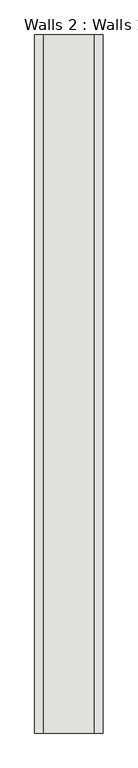
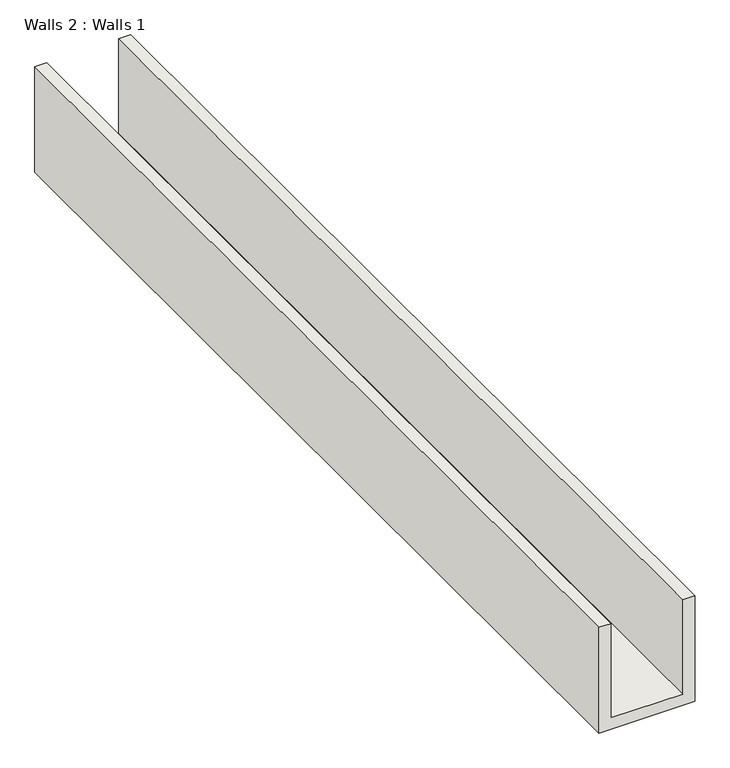
"""IFC4 building model written with IfcOpenShell, lengths in millimetres: wall geometry, Walls 2 : Walls 1."""

from ifc_helpers import new_model, si_unit, frame, origin, place, context, project, spatial, polyline, outline, extrude, source, transform, mapped, element, save


def walls_2_walls_1_c83e6538(model_context):
    return source(origin(), model_context, "Body", "SweptSolid", [
        extrude(outline(polyline([(2794.0, -1677.3168771), (3149.6, -1677.3168771), (3149.6, -1715.4168771), (2832.1, -1715.4168771), (2832.1, -1944.0168771), (3149.6, -1944.0168771), (3149.6, -1982.1168771), (2794.0, -1982.1168771), (2794.0, -1677.3168771)])), frame((0.0, -3023.5771465, 0.0), z_axis=(0.0, 1.0, 0.0), x_axis=(0.0, 0.0, 1.0)), (0.0, 0.0, 1.0), 3114.7191067),
    ])


if __name__ == "__main__":
    model = new_model("IFC4")
    model_context = context("Model", 3, world=origin())
    ifc_project = project(units=[si_unit("LENGTHUNIT", "METRE", prefix="MILLI")], contexts=[model_context])
    site = spatial("IfcSite", under=ifc_project)
    building = spatial("IfcBuilding", under=site)
    placement = place(None, origin())
    walls_2_walls_1_shape = walls_2_walls_1_c83e6538(model_context)
    element("IfcWall", 1, ObjectType="Walls 2 : Walls 1", at=placement, inside=building, context=model_context, shape_type="MappedRepresentation", body=[
        mapped(walls_2_walls_1_shape, transform((0.0, 0.0, 0.0), x_axis=(1.0, 0.0, 0.0), y_axis=(0.0, 1.0, 0.0), z_axis=(0.0, 0.0, 1.0))),
    ])
    save(model, "model.ifc")

# Revit data of these elements
# Element 1 (IfcWall, "Walls 2 : Walls 1")
#   Materials on its faces: "Stucco - Plaster Cement - Red"
# Materials
#   "Stucco - Plaster Cement - Red": class "Generic", colour RGB 127 70 82, transparency 0, Description = "Gypsum Wall Board", Cost = 0
